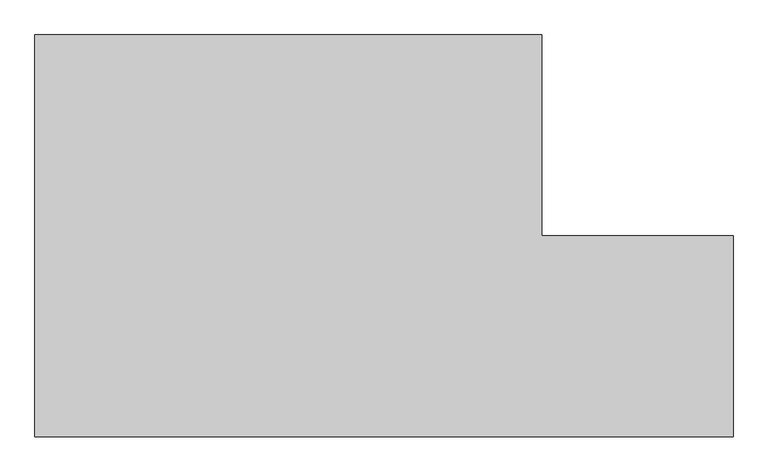
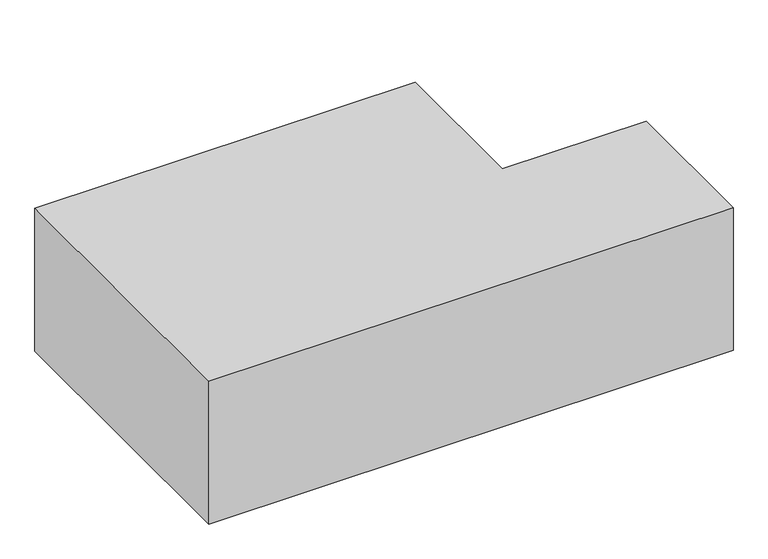
"""IFC4 building model written with IfcOpenShell, lengths in millimetres: proxy geometry, Приточная установка_П1 : СКВ ВОХ 10/10."""

from ifc_helpers import new_model, si_unit, origin, origin_with_axes, place, context, project, spatial, polyline, outline, extrude, source, transform, mapped, element, save


def mechanical_equipment_2ae54859(model_context):
    return source(origin(), model_context, "Body", "SweptSolid", [
        extrude(outline(polyline([(3650.0, 0.0), (0.0, 0.0), (0.0, 2100.0), (2650.0, 2100.0), (2650.0, 1050.0), (3650.0, 1050.0), (3650.0, 0.0)])), origin_with_axes(), (0.0, 0.0, 1.0), 1050.0),
    ])


if __name__ == "__main__":
    model = new_model("IFC4")
    model_context = context("Model", 3, world=origin())
    ifc_project = project(units=[si_unit("LENGTHUNIT", "METRE", prefix="MILLI")], contexts=[model_context])
    site = spatial("IfcSite", under=ifc_project)
    building = spatial("IfcBuilding", under=site)
    placement = place(None, origin())
    mechanical_equipment_shape = mechanical_equipment_2ae54859(model_context)
    element("IfcBuildingElementProxy", 1, Name="Приточная установка_П1 : СКВ ВОХ 10/10", ObjectType="Приточная установка_П1 : СКВ ВОХ 10/10", at=placement, inside=building, context=model_context, shape_type="MappedRepresentation", body=[
        mapped(mechanical_equipment_shape, transform((0.0, 0.0, 0.0), x_axis=(1.0, 0.0, 0.0), y_axis=(0.0, 1.0, 0.0), z_axis=(0.0, 0.0, 1.0))),
    ])
    save(model, "model.ifc")

# Revit data of these elements
# Type "Приточная установка_П1 : СКВ ВОХ 10/10"
#   ADSK_Позиция = "20"
#   ADSK_Наименование = "Установка приточная"
#   ADSK_Марка = "СКВ ВОХ 10/1О-S-35,TY 4862-001-22330703-2014 комплектация по обосновывающему документу 0092.020.013.Р4. 0004.653.0000.3502 .003-08.ОЛ1 инв.№10041700, 0092.020.013.Р4. 0004.653.0000.3502 .003-ОВ.Н1 инв. №10041709"
#   ADSK_Код изделия = "4261596"
#   ADSK_Завод-изготовитель = "ООО \"АЭРО ИКСИА\", Россия, г. Брянск, ИНН 3257017280, КП П 5261 О 1001, aero@ixia.su"
#   ADSK_Единица измерения = "компл."
#   Ширина соединения = 900 mm
#   Ширина приточной части = 1050 mm
#   Ширина = 3650 mm
#   Подключение к теплосети = 65 mm
#   Длина = 2100 mm
#   Высота соединения = 900 mm
#   Высота = 1050 mm
#   ADSK_Масса = 1091
#   ADSK_Количество = 1
#   Default Elevation = 0
